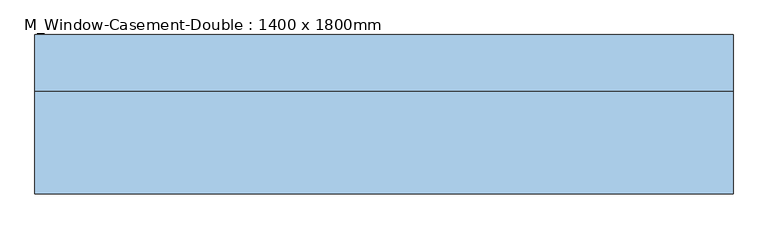
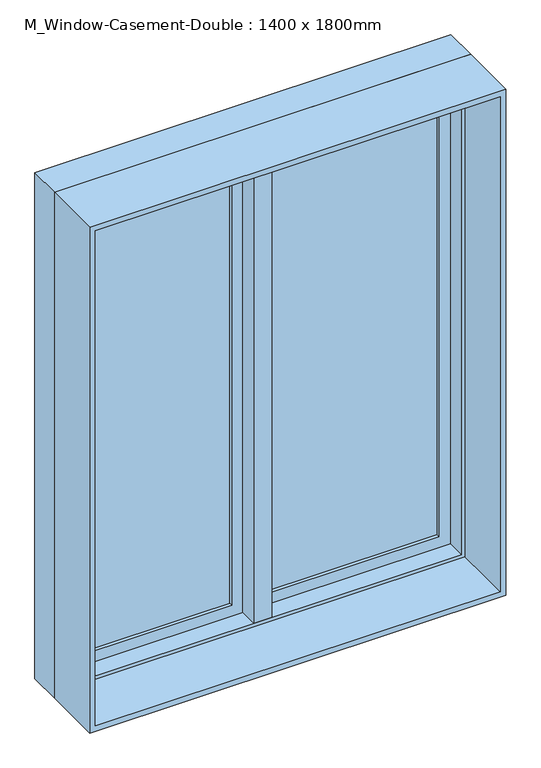
"""IFC4 building model written with IfcOpenShell, lengths in millimetres: window geometry, M_Window-Casement-Double : 1400 x 1800mm."""

from ifc_helpers import new_model, si_unit, frame, origin, place, context, project, spatial, polyline, outline, extrude, faceted_brep, source, transform, mapped, element, save


def m_window_casement_double_1400_x_1800mm_f8d7c7c6(model_context):
    return source(origin(), model_context, "Body", "SolidModel", [
        faceted_brep([(9.525, 169.05, 2687.3), (-9.525, 169.05, 2687.3), (-9.525, 118.25, 2687.3), (9.525, 118.25, 2687.3), (9.525, 169.05, 912.7), (9.525, 118.25, 912.7), (-9.525, 118.25, 912.7), (-9.525, 169.05, 912.7), (-9.525, 118.25, 931.75), (-9.525, 118.25, 2668.25), (-30.1625, 118.25, 931.75), (-30.1625, 118.25, 2668.25), (-30.1625, 54.75, 931.75), (-30.1625, 54.75, 2668.25), (30.1625, 54.75, 931.75), (30.1625, 54.75, 2668.25), (30.1625, 118.25, 931.75), (30.1625, 118.25, 2668.25), (9.525, 118.25, 931.75), (9.525, 118.25, 2668.25)], [[[0, 1, 2, 3]], [[4, 5, 6, 7]], [[1, 0, 4, 7]], [[2, 1, 7, 6, 8, 9]], [[9, 8, 10, 11]], [[11, 10, 12, 13]], [[13, 12, 14, 15]], [[15, 14, 16, 17]], [[17, 16, 18, 19]], [[0, 3, 19, 18, 5, 4]], [[18, 8, 6, 5]], [[9, 19, 3, 2]], [[8, 18, 16, 14, 12, 10]], [[19, 9, 11, 13, 15, 17]]]),
        extrude(outline(polyline([(-66.675, 150.0), (-66.675, 143.65), (-630.15, 143.65), (-630.15, 150.0), (-66.675, 150.0)])), frame((0.0, 0.0, 969.85), z_axis=(0.0, 0.0, 1.0), x_axis=(1.0, 0.0, 0.0)), (0.0, 0.0, 1.0), 1660.3),
        extrude(outline(polyline([(-630.15, 130.95), (-630.15, 137.3), (-66.675, 137.3), (-66.675, 130.95), (-630.15, 130.95)])), frame((0.0, 0.0, 969.85), z_axis=(0.0, 0.0, 1.0), x_axis=(1.0, 0.0, 0.0)), (0.0, 0.0, 1.0), 1660.3),
        extrude(outline(polyline([(630.15, 150.0), (630.15, 143.65), (66.675, 143.65), (66.675, 150.0), (630.15, 150.0)])), frame((0.0, 0.0, 969.85), z_axis=(0.0, 0.0, 1.0), x_axis=(1.0, 0.0, 0.0)), (0.0, 0.0, 1.0), 1660.3),
        extrude(outline(polyline([(66.675, 130.95), (66.675, 137.3), (630.15, 137.3), (630.15, 130.95), (66.675, 130.95)])), frame((0.0, 0.0, 969.85), z_axis=(0.0, 0.0, 1.0), x_axis=(1.0, 0.0, 0.0)), (0.0, 0.0, 1.0), 1660.3),
        extrude(outline(polyline([(2687.3, -687.3), (912.7, -687.3), (912.7, -9.525), (2687.3, -9.525), (2687.3, -687.3)]), holes=[polyline([(2630.15, -66.675), (969.85, -66.675), (969.85, -630.15), (2630.15, -630.15), (2630.15, -66.675)])]), frame((0.0, 118.25, 0.0), z_axis=(0.0, 1.0, 0.0), x_axis=(0.0, 0.0, 1.0)), (0.0, 0.0, 1.0), 44.45),
        extrude(outline(polyline([(912.7, 687.3), (2687.3, 687.3), (2687.3, 9.525), (912.7, 9.525), (912.7, 687.3)]), holes=[polyline([(969.85, 66.675), (2630.15, 66.675), (2630.15, 630.15), (969.85, 630.15), (969.85, 66.675)])]), frame((0.0, 118.25, 0.0), z_axis=(0.0, 1.0, 0.0), x_axis=(0.0, 0.0, 1.0)), (0.0, 0.0, 1.0), 44.45),
        extrude(outline(polyline([(2700.0, -700.0), (900.0, -700.0), (900.0, 700.0), (2700.0, 700.0), (2700.0, -700.0)]), holes=[polyline([(2680.95, 680.95), (919.05, 680.95), (919.05, -680.95), (2680.95, -680.95), (2680.95, 680.95)])]), frame((0.0, -150.0, 0.0), z_axis=(0.0, 1.0, 0.0), x_axis=(0.0, 0.0, 1.0)), (0.0, 0.0, 1.0), 204.75),
        faceted_brep([(668.25, 118.25, 2668.25), (668.25, 54.75, 2668.25), (-668.25, 54.75, 2668.25), (-668.25, 118.25, 2668.25), (687.3, 169.05, 2687.3), (687.3, 118.25, 2687.3), (-687.3, 118.25, 2687.3), (-687.3, 169.05, 2687.3), (700.0, 54.75, 2700.0), (700.0, 169.05, 2700.0), (-700.0, 169.05, 2700.0), (-700.0, 54.75, 2700.0), (-668.25, 54.75, 931.75), (-668.25, 118.25, 931.75), (-687.3, 118.25, 912.7), (-687.3, 169.05, 912.7), (-700.0, 169.05, 900.0), (-700.0, 54.75, 900.0), (668.25, 54.75, 931.75), (668.25, 118.25, 931.75), (687.3, 118.25, 912.7), (687.3, 169.05, 912.7), (700.0, 169.05, 900.0), (700.0, 54.75, 900.0)], [[[0, 1, 2, 3]], [[4, 5, 6, 7]], [[8, 9, 10, 11]], [[3, 2, 12, 13]], [[7, 6, 14, 15]], [[11, 10, 16, 17]], [[13, 12, 18, 19]], [[15, 14, 20, 21]], [[17, 16, 22, 23]], [[11, 17, 23, 8], [1, 18, 12, 2]], [[19, 18, 1, 0]], [[5, 20, 14, 6], [3, 13, 19, 0]], [[21, 20, 5, 4]], [[23, 22, 9, 8]], [[9, 22, 16, 10], [7, 15, 21, 4]]]),
    ])


if __name__ == "__main__":
    model = new_model("IFC4")
    model_context = context("Model", 3, world=origin())
    ifc_project = project(units=[si_unit("LENGTHUNIT", "METRE", prefix="MILLI")], contexts=[model_context])
    site = spatial("IfcSite", under=ifc_project)
    building = spatial("IfcBuilding", under=site)
    placement = place(None, origin())
    m_window_casement_double_1400_x_1800mm_shape = m_window_casement_double_1400_x_1800mm_f8d7c7c6(model_context)
    element("IfcWindow", 1, ObjectType="M_Window-Casement-Double : 1400 x 1800mm", at=placement, inside=building, context=model_context, shape_type="MappedRepresentation", body=[
        mapped(m_window_casement_double_1400_x_1800mm_shape, transform((0.0, 0.0, 0.0), x_axis=(1.0, 0.0, 0.0), y_axis=(0.0, 1.0, 0.0), z_axis=(0.0, 0.0, 1.0))),
    ])
    save(model, "model.ifc")

# Revit data of these elements
# Type "M_Window-Casement-Double : 1400 x 1800mm"
#   Type Mark = "26"
#   Fire Rating = "0.5h"
#   Assembly Code = "B2020100"
#   Analytic Construction = "Double glazing - domestic"
#   Frame Extension [instance default] = 6.35 mm
#   Window Inset [instance default] = 0 mm
#   Wall Thickness [instance default] = 150 mm
#   Interior Wall Closure [instance default] = 54.75 mm
#   Half Width = 700 mm
#   Visual Light Transmittance = 0.81
#   Thermal Resistance (R) = 0.319569 (m²·K)/W
#   Solar Heat Gain Coefficient = 0.76
#   Rough Width = 1415 mm
#   Rough Height = 1815 mm
#   Height = 1800 mm
#   Heat Transfer Coefficient (U) = 3.12929 W/(m²·K)
#   Exterior Wall Closure [instance default] = 31.8 mm
#   Extension Jamb [instance default] = 54.75 mm
#   Default Sill Height = 900 mm
#   Width = 1400 mm
#   Define Thermal Properties by = 0
#   Muntin Visibility = yes
#   Interior Trim Visibility [instance default] = yes
#   Exterior Trim Visibility [instance default] = yes
#   Extension Jamb Visibility [instance default] = yes
#   Interior Trim Material = Wood - Stained
#   Muntin Pattern = M_Muntin Pattern_2x2 : M_Muntin Pattern_2x2
#   Interior Trim = M_Trim-Window-Interior-Flat : Picture Frame
#   Interior Frame Material = Wood - Stained
#   Glass Panel Material = Glass
#   Exterior Trim Material = Clad - White
#   Exterior Trim = M_Trim-Window-Exterior-Flat : with Sill
#   Exterior Frame Material = Clad - White
#   Wall Closure = (empty or 0)
# Element 1 (IfcWindow, "M_Window-Casement-Double : 1400 x 1800mm")
#   Wall Thickness = 300 mm
#   Extension Jamb = 204.75 mm
#   Materials on its faces: "Wood - Stained", "Glass", "Clad - White"
# Materials
#   "Wood - Stained": class "Wood", colour RGB 224 178 126, transparency 0, Cost = 0
#   "Glass": class "Glass", colour RGB 0 128 192, transparency 0.9, Description = "Soda Lime Glass", Cost = 0
#   "Clad - White": class "Wood", colour RGB 242 242 238, transparency 0, Cost = 0
